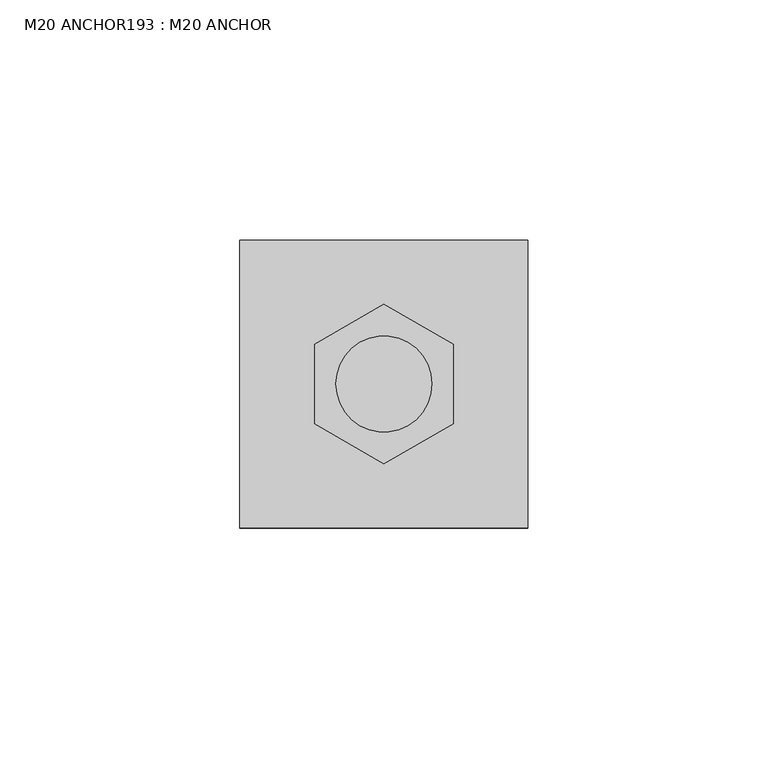
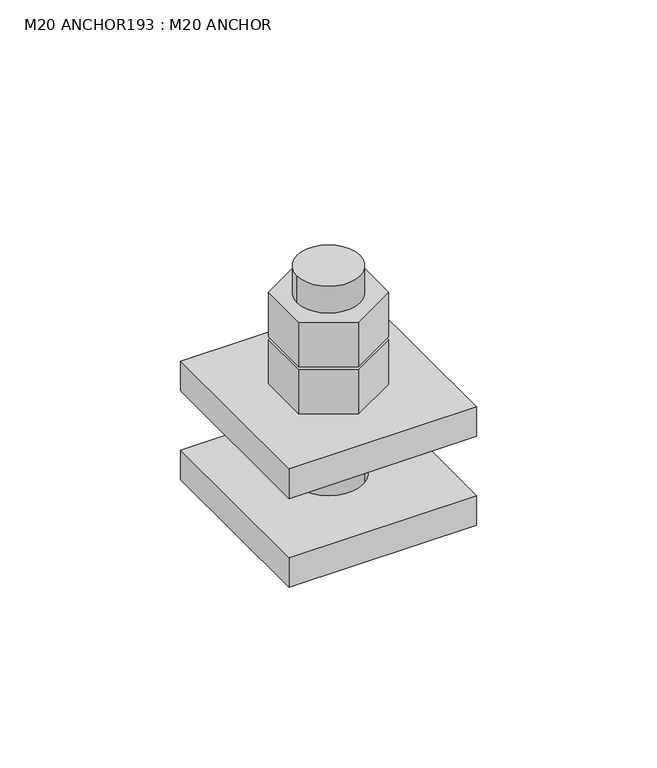
"""IFC4 building model written with IfcOpenShell, lengths in millimetres: fastener geometry, M20 ANCHOR193 : M20 ANCHOR."""

import ifcopenshell
import ifcopenshell.guid

model = None  # the IFC model being written
_history = None  # IfcOwnerHistory: only IFC2X3 demands one
_inside = {}  # id of a spatial element -> (the spatial element, [elements in it])
_under = {}  # id of a project, library or spatial element -> (it, [spatial elements below it])
_declared = {}  # id of a project -> (the project, [libraries it declares])
_typed = {}  # id of a type object -> (the type object, [elements of that type])
_made_of = {}  # id of a material, layer set ... -> (it, [elements and type objects made of it])


def new_model(schema):
    """Start an empty IFC model of exactly this schema.

    Asked for "IFC4X3", IfcOpenShell would pick the latest addendum, in which some entities
    have other attributes; the version numbers below select the first issue.
    IFC2X3 requires an IfcOwnerHistory on every rooted entity: one is made here for all.
    """
    global model, _history
    if schema == "IFC4X3":
        model = ifcopenshell.file(schema_version=(4, 3, 0, 0))
    else:
        model = ifcopenshell.file(schema=schema)
    _inside.clear()
    _under.clear()
    _declared.clear()
    _typed.clear()
    _made_of.clear()
    _history = None
    if model.schema == "IFC2X3":
        org = make("IfcOrganization", Name="unknown")
        user = make(
            "IfcPersonAndOrganization",
            ThePerson=make("IfcPerson", FamilyName="unknown"),
            TheOrganization=org,
        )
        app = make(
            "IfcApplication",
            ApplicationDeveloper=org,
            Version="unknown",
            ApplicationFullName="unknown",
            ApplicationIdentifier="unknown",
        )
        _history = make(
            "IfcOwnerHistory",
            OwningUser=user,
            OwningApplication=app,
            ChangeAction="ADDED",
            CreationDate=0,
        )
    return model


def make(cls, **values):
    """One entity of the class cls with the attributes given. An attribute that is None is left unset."""
    return model.create_entity(
        cls, **{name: value for name, value in values.items() if value is not None}
    )


def rooted(cls, **values):
    """An entity with a GlobalId (a new one), such as an element, a storey or a relation."""
    return make(cls, GlobalId=ifcopenshell.guid.new(), OwnerHistory=_history, **values)


def si_unit(unit_type, name, prefix=None):
    """IfcSIUnit, for example si_unit("LENGTHUNIT", "METRE", prefix="MILLI")."""
    return make("IfcSIUnit", UnitType=unit_type, Prefix=prefix, Name=name)


def assignment(units):
    """IfcUnitAssignment: the units of a project."""
    return None if units is None else make("IfcUnitAssignment", Units=units)


def point(xyz):
    """IfcCartesianPoint."""
    return None if xyz is None else make("IfcCartesianPoint", Coordinates=xyz)


def direction(xyz):
    """IfcDirection."""
    return None if xyz is None else make("IfcDirection", DirectionRatios=xyz)


def frame(location, z_axis=None, x_axis=None):
    """IfcAxis2Placement3D, a coordinate frame: its origin and axes. An axis left out is left unset."""
    return make(
        "IfcAxis2Placement3D",
        Location=point(location),
        Axis=direction(z_axis),
        RefDirection=direction(x_axis),
    )


def frame_2d(location, x_axis=None):
    """IfcAxis2Placement2D, a coordinate frame in the plane: its origin and x axis."""
    return make(
        "IfcAxis2Placement2D", Location=point(location), RefDirection=direction(x_axis)
    )


def origin():
    """The frame at (0, 0, 0) with its axes left unset."""
    return frame((0.0, 0.0, 0.0))


def place(relative_to, where):
    """IfcLocalPlacement: puts the frame where relative to a parent placement (None: the world)."""
    return make(
        "IfcLocalPlacement", PlacementRelTo=relative_to, RelativePlacement=where
    )


def context(
    kind, dimensions, precision=None, world=None, true_north=None, identifier=None
):
    """IfcGeometricRepresentationContext, for example the 3D "Model" context."""
    return make(
        "IfcGeometricRepresentationContext",
        ContextIdentifier=identifier,
        ContextType=kind,
        CoordinateSpaceDimension=dimensions,
        Precision=precision,
        WorldCoordinateSystem=world,
        TrueNorth=true_north,
    )


def project(units=None, contexts=None):
    """IfcProject with its units and contexts."""
    return rooted(
        "IfcProject",
        Name="project",
        RepresentationContexts=contexts,
        UnitsInContext=assignment(units),
    )


def spatial(cls, under=None, at=None, **own):
    """A site, building, storey or space (cls), placed at a placement, below another one or the project."""
    s = rooted(cls, ObjectPlacement=at, **own)
    if under is not None:
        _under.setdefault(under.id(), (under, []))[1].append(s)
    return s


def polyline(points):
    """IfcPolyline through the points."""
    return make("IfcPolyline", Points=[point(p) for p in points])


def circle_curve(where, radius):
    """IfcCircle in the frame where."""
    return make("IfcCircle", Position=where, Radius=radius)


def trimmed(basis, trim1, trim2, sense, master):
    """IfcTrimmedCurve: the piece of a basis curve between two trims."""
    return make(
        "IfcTrimmedCurve",
        BasisCurve=basis,
        Trim1=trim1,
        Trim2=trim2,
        SenseAgreement=sense,
        MasterRepresentation=master,
    )


def segment(curve, same_sense, transition):
    """IfcCompositeCurveSegment."""
    return make(
        "IfcCompositeCurveSegment",
        Transition=transition,
        SameSense=same_sense,
        ParentCurve=curve,
    )


def composite_curve(segments, self_intersect=None):
    """IfcCompositeCurve: segments joined end to end."""
    return make("IfcCompositeCurve", Segments=segments, SelfIntersect=self_intersect)


def outline(outer, holes=None, kind="AREA"):
    """IfcArbitraryClosedProfileDef: a profile drawn as a closed curve; with holes, ...WithVoids."""
    if holes is None:
        return make("IfcArbitraryClosedProfileDef", ProfileType=kind, OuterCurve=outer)
    return make(
        "IfcArbitraryProfileDefWithVoids",
        ProfileType=kind,
        OuterCurve=outer,
        InnerCurves=holes,
    )


def extrude(swept, where, along, depth):
    """IfcExtrudedAreaSolid: the profile swept, set in the frame where, extruded along a direction by depth."""
    return make(
        "IfcExtrudedAreaSolid",
        SweptArea=swept,
        Position=where,
        ExtrudedDirection=direction(along),
        Depth=depth,
    )


def shape(context_of_items, identifier, shape_type, items):
    """IfcShapeRepresentation: the items that make up one representation, for example the "Body"."""
    return make(
        "IfcShapeRepresentation",
        ContextOfItems=context_of_items,
        RepresentationIdentifier=identifier,
        RepresentationType=shape_type,
        Items=items,
    )


def source(mapping_origin, context_of_items, identifier, shape_type, items):
    """IfcRepresentationMap: a shape defined once, which mapped items show again and again."""
    return make(
        "IfcRepresentationMap",
        MappingOrigin=mapping_origin,
        MappedRepresentation=shape(context_of_items, identifier, shape_type, items),
    )


def transform(
    local_origin,
    x_axis=None,
    y_axis=None,
    z_axis=None,
    scale=None,
    scale2=None,
    scale3=None,
    uniform=True,
):
    """IfcCartesianTransformationOperator3D, or its non-uniform kind. x_axis, y_axis, z_axis: its Axis1, 2, 3."""
    if uniform:
        return make(
            "IfcCartesianTransformationOperator3D",
            Axis1=direction(x_axis),
            Axis2=direction(y_axis),
            LocalOrigin=point(local_origin),
            Scale=scale,
            Axis3=direction(z_axis),
        )
    return make(
        "IfcCartesianTransformationOperator3DnonUniform",
        Axis1=direction(x_axis),
        Axis2=direction(y_axis),
        LocalOrigin=point(local_origin),
        Scale=scale,
        Axis3=direction(z_axis),
        Scale2=scale2,
        Scale3=scale3,
    )


def mapped(mapping_source, mapping_target):
    """IfcMappedItem: shows the shape of a source again, moved by a transform."""
    return make(
        "IfcMappedItem", MappingSource=mapping_source, MappingTarget=mapping_target
    )


def made_of(thing, what):
    """Note that an element or type object is made of a material, layer set ...; save() writes the relation."""
    if what is not None:
        _made_of.setdefault(what.id(), (what, []))[1].append(thing)
    return thing


def element(
    cls,
    number,
    at=None,
    inside=None,
    cuts=None,
    type_object=None,
    material=None,
    context=None,
    identifier="Body",
    shape_type=None,
    held_by="IfcProductDefinitionShape",
    body=None,
    shapes=None,
    **own,
):
    """One element of the class cls, such as IfcWall. Its Tag is "e" and its number.

    at: its placement. inside: the storey or other place that contains it. cuts: it is an
    opening in that element (IfcRelVoidsElement). A single representation is given by context,
    identifier, shape_type and body (its items); several are given by shapes. held_by: the class
    of the entity that holds the representations. save() writes the other relations.
    """
    e = rooted(cls, Tag="e%d" % number, ObjectPlacement=at, **own)
    if body is not None:
        shapes = [shape(context, identifier, shape_type, body)]
    if shapes is not None:
        e.Representation = make(held_by, Representations=shapes)
    if inside is not None:
        _inside.setdefault(inside.id(), (inside, []))[1].append(e)
    if cuts is not None:
        rooted(
            "IfcRelVoidsElement", RelatingBuildingElement=cuts, RelatedOpeningElement=e
        )
    if type_object is not None:
        _typed.setdefault(type_object.id(), (type_object, []))[1].append(e)
    return made_of(e, material)


def aggregate(whole, parts):
    """IfcRelAggregates: a whole, such as a stair, and the parts it consists of."""
    return rooted("IfcRelAggregates", RelatingObject=whole, RelatedObjects=parts)


def save(model, path):
    """Write the relations noted so far, then the file.

    IfcRelAggregates (storeys below a building ...), IfcRelContainedInSpatialStructure (elements
    in a storey), IfcRelDefinesByType, IfcRelAssociatesMaterial and IfcRelDeclares: one each for
    every whole, place, type object, material and project.
    """
    for whole, parts in _under.values():
        aggregate(whole, parts)
    for where, things in _inside.values():
        rooted(
            "IfcRelContainedInSpatialStructure",
            RelatedElements=things,
            RelatingStructure=where,
        )
    for kind, things in _typed.values():
        rooted("IfcRelDefinesByType", RelatedObjects=things, RelatingType=kind)
    for what, things in _made_of.values():
        rooted("IfcRelAssociatesMaterial", RelatedObjects=things, RelatingMaterial=what)
    for by, libraries in _declared.values():
        rooted("IfcRelDeclares", RelatingContext=by, RelatedDefinitions=libraries)
    model.write(path)


def m20_anchor193_m20_anchor_e1222fd5(model_context):
    return source(origin(), model_context, "Body", "SweptSolid", [
        extrude(outline(polyline([(8991.9144032, 19453.9464399), (8977.5062842, 19445.6279085), (8963.0981652, 19453.9464399), (8963.0981652, 19470.5835027), (8977.5062842, 19478.9020341), (8991.9144032, 19470.5835027), (8991.9144032, 19453.9464399)]), holes=[composite_curve([segment(trimmed(circle_curve(frame_2d((8977.5062842, 19462.2649713)), 10.0), [point((8967.5062842, 19462.2649713))], [point((8987.5062842, 19462.2649713))], True, "CARTESIAN"), True, "CONTINUOUS"), segment(trimmed(circle_curve(frame_2d((8977.5062842, 19462.2649713)), 10.0), [point((8987.5062842, 19462.2649713))], [point((8967.5062842, 19462.2649713))], True, "CARTESIAN"), True, "CONTINUOUS")], self_intersect=False)]), frame((0.0, 0.0, 246.0), z_axis=(0.0, 0.0, 1.0), x_axis=(1.0, 0.0, 0.0)), (0.0, 0.0, 1.0), 15.0),
        extrude(outline(polyline([(8991.9144032, 19453.9464399), (8977.5062842, 19445.6279085), (8963.0981652, 19453.9464399), (8963.0981652, 19470.5835027), (8977.5062842, 19478.9020341), (8991.9144032, 19470.5835027), (8991.9144032, 19453.9464399)]), holes=[composite_curve([segment(trimmed(circle_curve(frame_2d((8977.5062842, 19462.2649713)), 10.0), [point((8967.5062842, 19462.2649713))], [point((8987.5062842, 19462.2649713))], True, "CARTESIAN"), True, "CONTINUOUS"), segment(trimmed(circle_curve(frame_2d((8977.5062842, 19462.2649713)), 10.0), [point((8987.5062842, 19462.2649713))], [point((8967.5062842, 19462.2649713))], True, "CARTESIAN"), True, "CONTINUOUS")], self_intersect=False)]), frame((0.0, 0.0, 230.0), z_axis=(0.0, 0.0, 1.0), x_axis=(1.0, 0.0, 0.0)), (0.0, 0.0, 1.0), 15.0),
        extrude(outline(composite_curve([segment(trimmed(circle_curve(frame_2d((8977.5062842, 19462.2649713)), 10.0), [point((8967.5062842, 19462.2649713))], [point((8987.5062842, 19462.2649713))], False, "CARTESIAN"), True, "CONTINUOUS"), segment(trimmed(circle_curve(frame_2d((8977.5062842, 19462.2649713)), 10.0), [point((8987.5062842, 19462.2649713))], [point((8967.5062842, 19462.2649713))], False, "CARTESIAN"), True, "CONTINUOUS")], self_intersect=False)), frame((0.0, 0.0, 190.0), z_axis=(0.0, 0.0, 1.0), x_axis=(1.0, 0.0, 0.0)), (0.0, 0.0, 1.0), 80.0),
        extrude(outline(polyline([(9007.5062842, 19432.2649713), (8947.5062842, 19432.2649713), (8947.5062842, 19492.2649713), (9007.5062842, 19492.2649713), (9007.5062842, 19432.2649713)]), holes=[composite_curve([segment(trimmed(circle_curve(frame_2d((8977.5062842, 19462.2649713)), 11.0), [point((8966.5062842, 19462.2649713))], [point((8988.5062842, 19462.2649713))], True, "CARTESIAN"), True, "CONTINUOUS"), segment(trimmed(circle_curve(frame_2d((8977.5062842, 19462.2649713)), 11.0), [point((8988.5062842, 19462.2649713))], [point((8966.5062842, 19462.2649713))], True, "CARTESIAN"), True, "CONTINUOUS")], self_intersect=False)]), frame((0.0, 0.0, 190.0), z_axis=(0.0, 0.0, 1.0), x_axis=(1.0, 0.0, 0.0)), (0.0, 0.0, 1.0), 10.0),
        extrude(outline(polyline([(9007.5062842, 19432.2649713), (8947.5062842, 19432.2649713), (8947.5062842, 19492.2649713), (9007.5062842, 19492.2649713), (9007.5062842, 19432.2649713)]), holes=[composite_curve([segment(trimmed(circle_curve(frame_2d((8977.5062842, 19462.2649713)), 11.0), [point((8966.5062842, 19462.2649713))], [point((8988.5062842, 19462.2649713))], True, "CARTESIAN"), True, "CONTINUOUS"), segment(trimmed(circle_curve(frame_2d((8977.5062842, 19462.2649713)), 11.0), [point((8988.5062842, 19462.2649713))], [point((8966.5062842, 19462.2649713))], True, "CARTESIAN"), True, "CONTINUOUS")], self_intersect=False)]), frame((0.0, 0.0, 220.0), z_axis=(0.0, 0.0, 1.0), x_axis=(1.0, 0.0, 0.0)), (0.0, 0.0, 1.0), 10.0),
    ])


if __name__ == "__main__":
    model = new_model("IFC4")
    model_context = context("Model", 3, world=origin())
    ifc_project = project(units=[si_unit("LENGTHUNIT", "METRE", prefix="MILLI")], contexts=[model_context])
    site = spatial("IfcSite", under=ifc_project)
    building = spatial("IfcBuilding", under=site)
    placement = place(None, origin())
    m20_anchor193_m20_anchor_shape = m20_anchor193_m20_anchor_e1222fd5(model_context)
    element("IfcFastener", 1, ObjectType="M20 ANCHOR193 : M20 ANCHOR", at=placement, inside=building, context=model_context, shape_type="MappedRepresentation", body=[
        mapped(m20_anchor193_m20_anchor_shape, transform((0.0, 0.0, 0.0), x_axis=(1.0, 0.0, 0.0), y_axis=(0.0, 1.0, 0.0), z_axis=(0.0, 0.0, 1.0))),
    ])
    save(model, "model.ifc")
